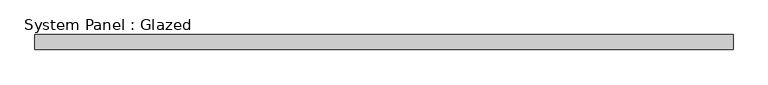
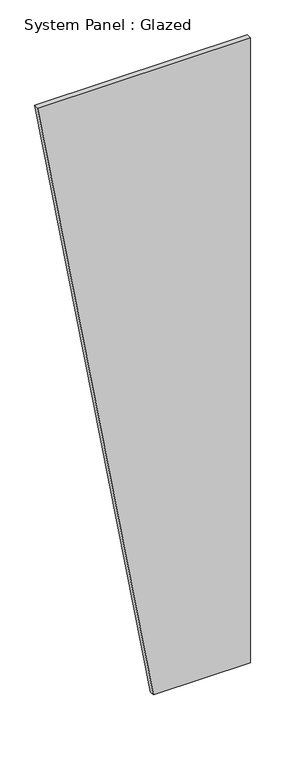
"""IFC4 building model written with IfcOpenShell, lengths in millimetres: plate geometry, System Panel : Glazed."""

from ifc_helpers import new_model, si_unit, frame, origin, place, context, project, spatial, polyline, outline, extrude, source, transform, mapped, element, save


def system_panel_glazed_bcd6892e(model_context):
    return source(origin(), model_context, "Body", "SweptSolid", [
        extrude(outline(polyline([(0.0, 53.0003468), (0.0, 589.4790509), (3657.6, 589.4790509), (3657.6, -589.4790509), (0.0, 53.0003468)])), frame((0.0, -44.45, 0.0), z_axis=(0.0, 1.0, 0.0), x_axis=(0.0, 0.0, 1.0)), (0.0, 0.0, 1.0), 25.4),
    ])


if __name__ == "__main__":
    model = new_model("IFC4")
    model_context = context("Model", 3, world=origin())
    ifc_project = project(units=[si_unit("LENGTHUNIT", "METRE", prefix="MILLI")], contexts=[model_context])
    site = spatial("IfcSite", under=ifc_project)
    building = spatial("IfcBuilding", under=site)
    placement = place(None, origin())
    system_panel_glazed_shape = system_panel_glazed_bcd6892e(model_context)
    element("IfcPlate", 1, ObjectType="System Panel : Glazed", at=placement, inside=building, context=model_context, shape_type="MappedRepresentation", body=[
        mapped(system_panel_glazed_shape, transform((0.0, 0.0, 0.0), x_axis=(1.0, 0.0, 0.0), y_axis=(0.0, 1.0, 0.0), z_axis=(0.0, 0.0, 1.0))),
    ])
    save(model, "model.ifc")

# Revit data of these elements
# Type "System Panel : Glazed"
#   Construction Type Id = "GSP4R"
#   Analytic Construction = "1/8 in Pilkington single glazing"
#   Visual Light Transmittance = 0.9
#   Solar Heat Gain Coefficient = 0.86
#   Heat Transfer Coefficient (U) = 1.18115 BTU/(h·ft²·°F)
#   Define Thermal Properties by = 1
# Element 1 (IfcPlate, "System Panel : Glazed")
#   Materials on its faces: "Glass"
# Materials
#   "Glass": class "Glass", colour RGB 0 128 192, transparency 0.75, Description = "Soda Lime Glass", Cost = 0
